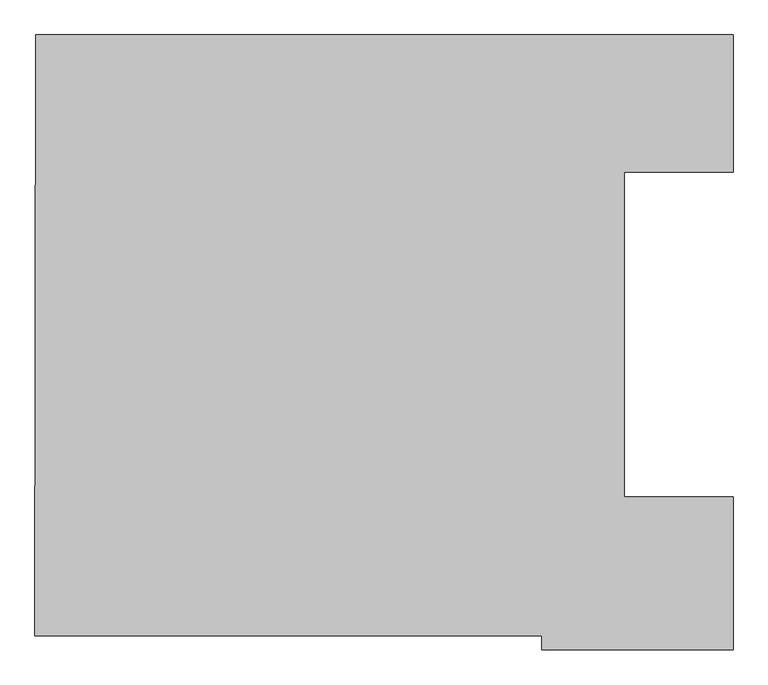
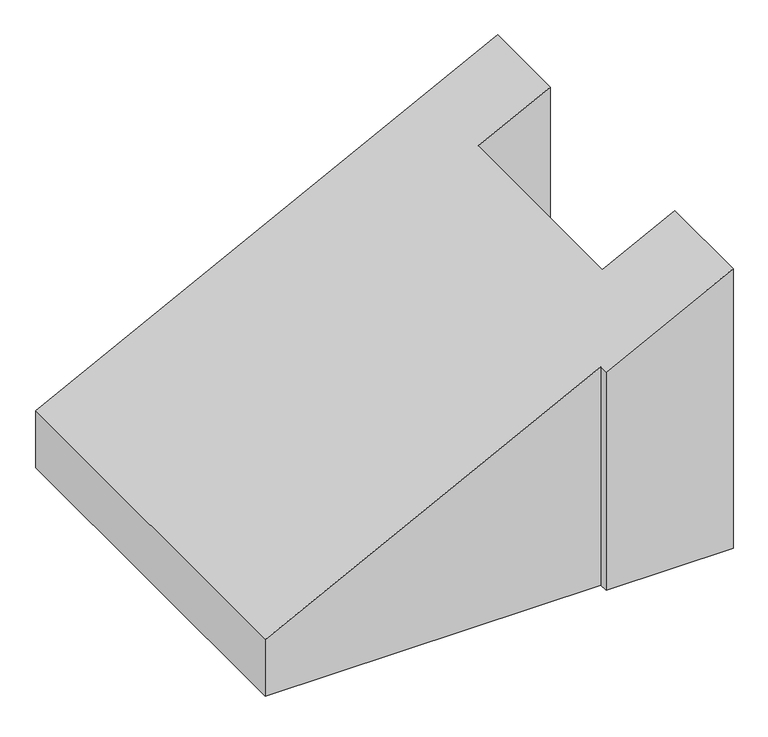
"""IFC4 building model written with IfcOpenShell, lengths in millimetres: proxy geometry, 0_3d_modell."""

from ifc_helpers import new_model, si_unit, origin, place, context, project, spatial, faceted_brep, source, transform, mapped, element, save


def generic_models_03464ee4(model_context):
    return source(origin(), model_context, "Body", "Brep", [
        faceted_brep([(4760.0, 130.0, 3273.5797924), (4760.0, 0.0, 3273.5797924), (6560.0, 0.0, 4190.7256015), (6560.0, 1435.0, 4190.7256015), (5535.0, 1435.0, 3668.4620158), (5535.0, 4487.8, 3668.4620158), (6560.0, 4487.8, 4190.7256015), (6560.0, 5780.0, 4190.7256015), (10.0, 5780.0, 853.3339073), (0.0, 130.0, 848.2386528), (5535.0, 4487.8, 0.0), (6560.0, 4487.8, 0.0), (5535.0, 1435.0, 0.0), (6560.0, 1435.0, 0.0), (4760.0, 0.0, 0.0), (6560.0, 0.0, 0.0), (4760.0, 130.0, 0.0), (0.0, 130.0, 0.0), (10.0, 5780.0, 0.0), (6560.0, 5780.0, 0.0)], [[[0, 1, 2, 3, 4, 5, 6, 7, 8, 9]], [[6, 5, 10, 11]], [[5, 4, 12, 10]], [[4, 3, 13, 12]], [[2, 1, 14, 15]], [[1, 0, 16, 14]], [[0, 9, 17, 16]], [[9, 8, 18, 17]], [[8, 7, 19, 18]], [[11, 19, 7, 6]], [[15, 13, 3, 2]], [[15, 14, 16, 17, 18, 19, 11, 10, 12, 13]]]),
    ])


if __name__ == "__main__":
    model = new_model("IFC4")
    model_context = context("Model", 3, world=origin())
    ifc_project = project(units=[si_unit("LENGTHUNIT", "METRE", prefix="MILLI")], contexts=[model_context])
    site = spatial("IfcSite", under=ifc_project)
    building = spatial("IfcBuilding", under=site)
    placement = place(None, origin())
    generic_models_shape = generic_models_03464ee4(model_context)
    element("IfcBuildingElementProxy", 1, Name="0_3d_modell", ObjectType="0_3d_modell", at=placement, inside=building, context=model_context, shape_type="MappedRepresentation", body=[
        mapped(generic_models_shape, transform((0.0, 0.0, 0.0), x_axis=(1.0, 0.0, 0.0), y_axis=(0.0, 1.0, 0.0), z_axis=(0.0, 0.0, 1.0))),
    ])
    save(model, "model.ifc")

# Revit data of these elements
# Element 1 (IfcBuildingElementProxy, "0_3d_modell")
#   Materials on its faces: "*1"
# Materials
#   "*1": class "Unassigned", colour RGB 175 175 175, transparency 0
